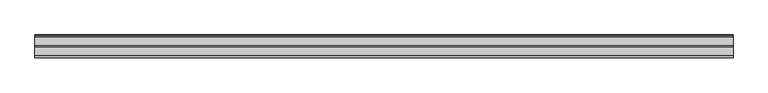
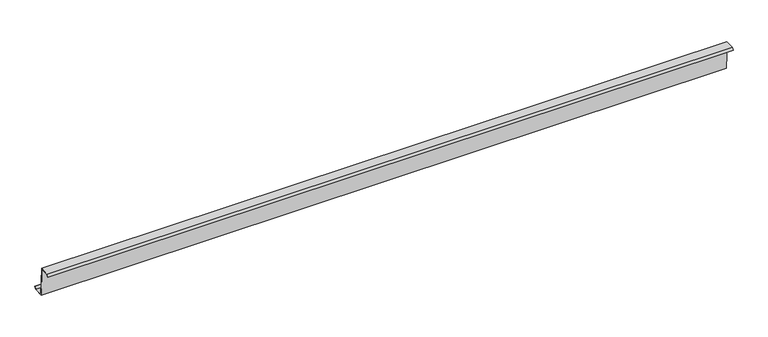
"""IFC4 building model written with IfcOpenShell, lengths in millimetres: proxy geometry, Generic Models 7:Generic Models 1:8:Generic Models 1:8 : Generic Models 7:Generic Models 1:337419:10 : Generic Models 7:Generic Models 1:8:Generic Models 1:8 : Generic Models 7:Generic Models 1:337419:315935."""

import ifcopenshell
import ifcopenshell.guid

model = None  # the IFC model being written
_history = None  # IfcOwnerHistory: only IFC2X3 demands one
_inside = {}  # id of a spatial element -> (the spatial element, [elements in it])
_under = {}  # id of a project, library or spatial element -> (it, [spatial elements below it])
_declared = {}  # id of a project -> (the project, [libraries it declares])
_typed = {}  # id of a type object -> (the type object, [elements of that type])
_made_of = {}  # id of a material, layer set ... -> (it, [elements and type objects made of it])


def new_model(schema):
    """Start an empty IFC model of exactly this schema.

    Asked for "IFC4X3", IfcOpenShell would pick the latest addendum, in which some entities
    have other attributes; the version numbers below select the first issue.
    IFC2X3 requires an IfcOwnerHistory on every rooted entity: one is made here for all.
    """
    global model, _history
    if schema == "IFC4X3":
        model = ifcopenshell.file(schema_version=(4, 3, 0, 0))
    else:
        model = ifcopenshell.file(schema=schema)
    _inside.clear()
    _under.clear()
    _declared.clear()
    _typed.clear()
    _made_of.clear()
    _history = None
    if model.schema == "IFC2X3":
        org = make("IfcOrganization", Name="unknown")
        user = make(
            "IfcPersonAndOrganization",
            ThePerson=make("IfcPerson", FamilyName="unknown"),
            TheOrganization=org,
        )
        app = make(
            "IfcApplication",
            ApplicationDeveloper=org,
            Version="unknown",
            ApplicationFullName="unknown",
            ApplicationIdentifier="unknown",
        )
        _history = make(
            "IfcOwnerHistory",
            OwningUser=user,
            OwningApplication=app,
            ChangeAction="ADDED",
            CreationDate=0,
        )
    return model


def make(cls, **values):
    """One entity of the class cls with the attributes given. An attribute that is None is left unset."""
    return model.create_entity(
        cls, **{name: value for name, value in values.items() if value is not None}
    )


def rooted(cls, **values):
    """An entity with a GlobalId (a new one), such as an element, a storey or a relation."""
    return make(cls, GlobalId=ifcopenshell.guid.new(), OwnerHistory=_history, **values)


def si_unit(unit_type, name, prefix=None):
    """IfcSIUnit, for example si_unit("LENGTHUNIT", "METRE", prefix="MILLI")."""
    return make("IfcSIUnit", UnitType=unit_type, Prefix=prefix, Name=name)


def assignment(units):
    """IfcUnitAssignment: the units of a project."""
    return None if units is None else make("IfcUnitAssignment", Units=units)


def point(xyz):
    """IfcCartesianPoint."""
    return None if xyz is None else make("IfcCartesianPoint", Coordinates=xyz)


def direction(xyz):
    """IfcDirection."""
    return None if xyz is None else make("IfcDirection", DirectionRatios=xyz)


def frame(location, z_axis=None, x_axis=None):
    """IfcAxis2Placement3D, a coordinate frame: its origin and axes. An axis left out is left unset."""
    return make(
        "IfcAxis2Placement3D",
        Location=point(location),
        Axis=direction(z_axis),
        RefDirection=direction(x_axis),
    )


def origin():
    """The frame at (0, 0, 0) with its axes left unset."""
    return frame((0.0, 0.0, 0.0))


def place(relative_to, where):
    """IfcLocalPlacement: puts the frame where relative to a parent placement (None: the world)."""
    return make(
        "IfcLocalPlacement", PlacementRelTo=relative_to, RelativePlacement=where
    )


def context(
    kind, dimensions, precision=None, world=None, true_north=None, identifier=None
):
    """IfcGeometricRepresentationContext, for example the 3D "Model" context."""
    return make(
        "IfcGeometricRepresentationContext",
        ContextIdentifier=identifier,
        ContextType=kind,
        CoordinateSpaceDimension=dimensions,
        Precision=precision,
        WorldCoordinateSystem=world,
        TrueNorth=true_north,
    )


def project(units=None, contexts=None):
    """IfcProject with its units and contexts."""
    return rooted(
        "IfcProject",
        Name="project",
        RepresentationContexts=contexts,
        UnitsInContext=assignment(units),
    )


def spatial(cls, under=None, at=None, **own):
    """A site, building, storey or space (cls), placed at a placement, below another one or the project."""
    s = rooted(cls, ObjectPlacement=at, **own)
    if under is not None:
        _under.setdefault(under.id(), (under, []))[1].append(s)
    return s


def polyline(points):
    """IfcPolyline through the points."""
    return make("IfcPolyline", Points=[point(p) for p in points])


def outline(outer, holes=None, kind="AREA"):
    """IfcArbitraryClosedProfileDef: a profile drawn as a closed curve; with holes, ...WithVoids."""
    if holes is None:
        return make("IfcArbitraryClosedProfileDef", ProfileType=kind, OuterCurve=outer)
    return make(
        "IfcArbitraryProfileDefWithVoids",
        ProfileType=kind,
        OuterCurve=outer,
        InnerCurves=holes,
    )


def extrude(swept, where, along, depth):
    """IfcExtrudedAreaSolid: the profile swept, set in the frame where, extruded along a direction by depth."""
    return make(
        "IfcExtrudedAreaSolid",
        SweptArea=swept,
        Position=where,
        ExtrudedDirection=direction(along),
        Depth=depth,
    )


def shape(context_of_items, identifier, shape_type, items):
    """IfcShapeRepresentation: the items that make up one representation, for example the "Body"."""
    return make(
        "IfcShapeRepresentation",
        ContextOfItems=context_of_items,
        RepresentationIdentifier=identifier,
        RepresentationType=shape_type,
        Items=items,
    )


def source(mapping_origin, context_of_items, identifier, shape_type, items):
    """IfcRepresentationMap: a shape defined once, which mapped items show again and again."""
    return make(
        "IfcRepresentationMap",
        MappingOrigin=mapping_origin,
        MappedRepresentation=shape(context_of_items, identifier, shape_type, items),
    )


def transform(
    local_origin,
    x_axis=None,
    y_axis=None,
    z_axis=None,
    scale=None,
    scale2=None,
    scale3=None,
    uniform=True,
):
    """IfcCartesianTransformationOperator3D, or its non-uniform kind. x_axis, y_axis, z_axis: its Axis1, 2, 3."""
    if uniform:
        return make(
            "IfcCartesianTransformationOperator3D",
            Axis1=direction(x_axis),
            Axis2=direction(y_axis),
            LocalOrigin=point(local_origin),
            Scale=scale,
            Axis3=direction(z_axis),
        )
    return make(
        "IfcCartesianTransformationOperator3DnonUniform",
        Axis1=direction(x_axis),
        Axis2=direction(y_axis),
        LocalOrigin=point(local_origin),
        Scale=scale,
        Axis3=direction(z_axis),
        Scale2=scale2,
        Scale3=scale3,
    )


def mapped(mapping_source, mapping_target):
    """IfcMappedItem: shows the shape of a source again, moved by a transform."""
    return make(
        "IfcMappedItem", MappingSource=mapping_source, MappingTarget=mapping_target
    )


def made_of(thing, what):
    """Note that an element or type object is made of a material, layer set ...; save() writes the relation."""
    if what is not None:
        _made_of.setdefault(what.id(), (what, []))[1].append(thing)
    return thing


def element(
    cls,
    number,
    at=None,
    inside=None,
    cuts=None,
    type_object=None,
    material=None,
    context=None,
    identifier="Body",
    shape_type=None,
    held_by="IfcProductDefinitionShape",
    body=None,
    shapes=None,
    **own,
):
    """One element of the class cls, such as IfcWall. Its Tag is "e" and its number.

    at: its placement. inside: the storey or other place that contains it. cuts: it is an
    opening in that element (IfcRelVoidsElement). A single representation is given by context,
    identifier, shape_type and body (its items); several are given by shapes. held_by: the class
    of the entity that holds the representations. save() writes the other relations.
    """
    e = rooted(cls, Tag="e%d" % number, ObjectPlacement=at, **own)
    if body is not None:
        shapes = [shape(context, identifier, shape_type, body)]
    if shapes is not None:
        e.Representation = make(held_by, Representations=shapes)
    if inside is not None:
        _inside.setdefault(inside.id(), (inside, []))[1].append(e)
    if cuts is not None:
        rooted(
            "IfcRelVoidsElement", RelatingBuildingElement=cuts, RelatedOpeningElement=e
        )
    if type_object is not None:
        _typed.setdefault(type_object.id(), (type_object, []))[1].append(e)
    return made_of(e, material)


def aggregate(whole, parts):
    """IfcRelAggregates: a whole, such as a stair, and the parts it consists of."""
    return rooted("IfcRelAggregates", RelatingObject=whole, RelatedObjects=parts)


def save(model, path):
    """Write the relations noted so far, then the file.

    IfcRelAggregates (storeys below a building ...), IfcRelContainedInSpatialStructure (elements
    in a storey), IfcRelDefinesByType, IfcRelAssociatesMaterial and IfcRelDeclares: one each for
    every whole, place, type object, material and project.
    """
    for whole, parts in _under.values():
        aggregate(whole, parts)
    for where, things in _inside.values():
        rooted(
            "IfcRelContainedInSpatialStructure",
            RelatedElements=things,
            RelatingStructure=where,
        )
    for kind, things in _typed.values():
        rooted("IfcRelDefinesByType", RelatedObjects=things, RelatingType=kind)
    for what, things in _made_of.values():
        rooted("IfcRelAssociatesMaterial", RelatedObjects=things, RelatingMaterial=what)
    for by, libraries in _declared.values():
        rooted("IfcRelDeclares", RelatingContext=by, RelatedDefinitions=libraries)
    model.write(path)


def generic_models_0f93359a(model_context):
    return source(origin(), model_context, "Body", "SweptSolid", [
        extrude(outline(polyline([(-565406.7257211, 8861.2163069), (-565341.8929127, 8863.917674), (-565333.5492409, 8663.6695501), (-565272.7864869, 8666.2013315), (-565261.9501902, 8680.2654109), (-565259.7495264, 8678.5698115), (-565271.3764942, 8663.4795457), (-565336.2093026, 8660.7781787), (-565344.5529744, 8861.0263025), (-565405.2854122, 8858.4957843), (-565416.1336128, 8844.4162551), (-565418.3526888, 8846.1260411), (-565406.7257211, 8861.2163069)])), frame((591306.0367242, 0.0, 0.0), z_axis=(1.0, 0.0, 0.0), x_axis=(0.0, 1.0, 0.0)), (0.0, 0.0, 1.0), 4876.8),
    ])


if __name__ == "__main__":
    model = new_model("IFC4")
    model_context = context("Model", 3, world=origin())
    ifc_project = project(units=[si_unit("LENGTHUNIT", "METRE", prefix="MILLI")], contexts=[model_context])
    site = spatial("IfcSite", under=ifc_project)
    building = spatial("IfcBuilding", under=site)
    placement = place(None, origin())
    generic_models_shape = generic_models_0f93359a(model_context)
    element("IfcBuildingElementProxy", 1, Name="Generic Models 7:Generic Models 1:8:Generic Models 1:8 : Generic Models 7:Generic Models 1:337419:10 : Generic Models 7:Generic Models 1:8:Generic Models 1:8 : Generic Models 7:Generic Models 1:337419:315935", ObjectType="Generic Models 7:Generic Models 1:8:Generic Models 1:8 : Generic Models 7:Generic Models 1:337419:10 : Generic Models 7:Generic Models 1:8:Generic Models 1:8 : Generic Models 7:Generic Models 1:337419:315935", at=placement, inside=building, context=model_context, shape_type="MappedRepresentation", body=[
        mapped(generic_models_shape, transform((0.0, 0.0, 0.0), x_axis=(1.0, 0.0, 0.0), y_axis=(0.0, 1.0, 0.0), z_axis=(0.0, 0.0, 1.0))),
    ])
    save(model, "model.ifc")

# Revit data of these elements
# Type "Generic Models 7:Generic Models 1:8:Generic Models 1:8 : Generic Models 7:Generic Models 1:337419:10 : Generic Models 7:Generic Models 1:8:Generic Models 1:8 : Generic Models 7:Generic Models 1:337419:315935"
#   NameOverride = "Generic Models 7:Generic Models 1:8:Generic Models 1:8 : Generic Models 7:Generic Models 1:337419:315935"
#   ObjectTypeOverride = "Generic Models 1:8 : Generic Models 7:Generic Models 1:337419"
#   Reference = "Generic Models 1"
#   Tag = "315935"
# Element 1 (IfcBuildingElementProxy, "Generic Models 7:Generic Models 1:8:Generic Models 1:8 : Generic Models 7:Generic Models 1:337419:10 : Generic Models 7:Generic Models 1:8:Generic Models 1:8 : Generic Models 7:Generic Models 1:337419:315935")
#   Materials on its faces: "ZEE' PURLIN (SEE STRUCT. DWGS)"
# Materials
#   "ZEE' PURLIN (SEE STRUCT. DWGS)": class "Unassigned", colour RGB 210 209 208, transparency 0, Cost = 0
